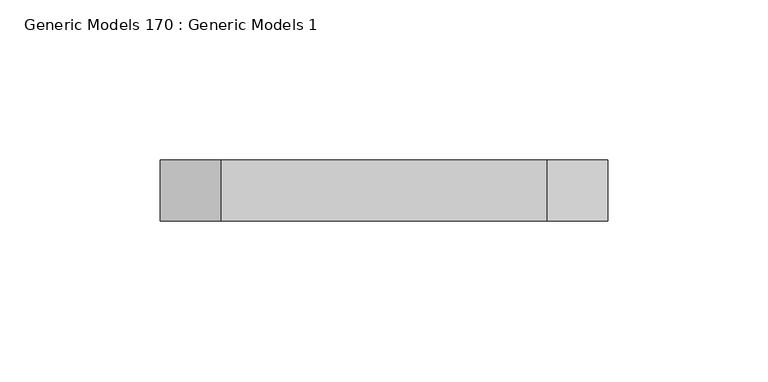
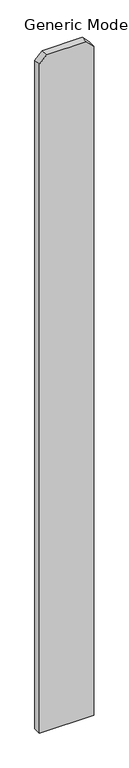
"""IFC4 building model written with IfcOpenShell, lengths in millimetres: proxy geometry, Generic Models 170 : Generic Models 1."""

import ifcopenshell
import ifcopenshell.guid

model = None  # the IFC model being written
_history = None  # IfcOwnerHistory: only IFC2X3 demands one
_inside = {}  # id of a spatial element -> (the spatial element, [elements in it])
_under = {}  # id of a project, library or spatial element -> (it, [spatial elements below it])
_declared = {}  # id of a project -> (the project, [libraries it declares])
_typed = {}  # id of a type object -> (the type object, [elements of that type])
_made_of = {}  # id of a material, layer set ... -> (it, [elements and type objects made of it])


def new_model(schema):
    """Start an empty IFC model of exactly this schema.

    Asked for "IFC4X3", IfcOpenShell would pick the latest addendum, in which some entities
    have other attributes; the version numbers below select the first issue.
    IFC2X3 requires an IfcOwnerHistory on every rooted entity: one is made here for all.
    """
    global model, _history
    if schema == "IFC4X3":
        model = ifcopenshell.file(schema_version=(4, 3, 0, 0))
    else:
        model = ifcopenshell.file(schema=schema)
    _inside.clear()
    _under.clear()
    _declared.clear()
    _typed.clear()
    _made_of.clear()
    _history = None
    if model.schema == "IFC2X3":
        org = make("IfcOrganization", Name="unknown")
        user = make(
            "IfcPersonAndOrganization",
            ThePerson=make("IfcPerson", FamilyName="unknown"),
            TheOrganization=org,
        )
        app = make(
            "IfcApplication",
            ApplicationDeveloper=org,
            Version="unknown",
            ApplicationFullName="unknown",
            ApplicationIdentifier="unknown",
        )
        _history = make(
            "IfcOwnerHistory",
            OwningUser=user,
            OwningApplication=app,
            ChangeAction="ADDED",
            CreationDate=0,
        )
    return model


def make(cls, **values):
    """One entity of the class cls with the attributes given. An attribute that is None is left unset."""
    return model.create_entity(
        cls, **{name: value for name, value in values.items() if value is not None}
    )


def rooted(cls, **values):
    """An entity with a GlobalId (a new one), such as an element, a storey or a relation."""
    return make(cls, GlobalId=ifcopenshell.guid.new(), OwnerHistory=_history, **values)


def si_unit(unit_type, name, prefix=None):
    """IfcSIUnit, for example si_unit("LENGTHUNIT", "METRE", prefix="MILLI")."""
    return make("IfcSIUnit", UnitType=unit_type, Prefix=prefix, Name=name)


def assignment(units):
    """IfcUnitAssignment: the units of a project."""
    return None if units is None else make("IfcUnitAssignment", Units=units)


def point(xyz):
    """IfcCartesianPoint."""
    return None if xyz is None else make("IfcCartesianPoint", Coordinates=xyz)


def direction(xyz):
    """IfcDirection."""
    return None if xyz is None else make("IfcDirection", DirectionRatios=xyz)


def frame(location, z_axis=None, x_axis=None):
    """IfcAxis2Placement3D, a coordinate frame: its origin and axes. An axis left out is left unset."""
    return make(
        "IfcAxis2Placement3D",
        Location=point(location),
        Axis=direction(z_axis),
        RefDirection=direction(x_axis),
    )


def origin():
    """The frame at (0, 0, 0) with its axes left unset."""
    return frame((0.0, 0.0, 0.0))


def place(relative_to, where):
    """IfcLocalPlacement: puts the frame where relative to a parent placement (None: the world)."""
    return make(
        "IfcLocalPlacement", PlacementRelTo=relative_to, RelativePlacement=where
    )


def context(
    kind, dimensions, precision=None, world=None, true_north=None, identifier=None
):
    """IfcGeometricRepresentationContext, for example the 3D "Model" context."""
    return make(
        "IfcGeometricRepresentationContext",
        ContextIdentifier=identifier,
        ContextType=kind,
        CoordinateSpaceDimension=dimensions,
        Precision=precision,
        WorldCoordinateSystem=world,
        TrueNorth=true_north,
    )


def project(units=None, contexts=None):
    """IfcProject with its units and contexts."""
    return rooted(
        "IfcProject",
        Name="project",
        RepresentationContexts=contexts,
        UnitsInContext=assignment(units),
    )


def spatial(cls, under=None, at=None, **own):
    """A site, building, storey or space (cls), placed at a placement, below another one or the project."""
    s = rooted(cls, ObjectPlacement=at, **own)
    if under is not None:
        _under.setdefault(under.id(), (under, []))[1].append(s)
    return s


def polyline(points):
    """IfcPolyline through the points."""
    return make("IfcPolyline", Points=[point(p) for p in points])


def outline(outer, holes=None, kind="AREA"):
    """IfcArbitraryClosedProfileDef: a profile drawn as a closed curve; with holes, ...WithVoids."""
    if holes is None:
        return make("IfcArbitraryClosedProfileDef", ProfileType=kind, OuterCurve=outer)
    return make(
        "IfcArbitraryProfileDefWithVoids",
        ProfileType=kind,
        OuterCurve=outer,
        InnerCurves=holes,
    )


def extrude(swept, where, along, depth):
    """IfcExtrudedAreaSolid: the profile swept, set in the frame where, extruded along a direction by depth."""
    return make(
        "IfcExtrudedAreaSolid",
        SweptArea=swept,
        Position=where,
        ExtrudedDirection=direction(along),
        Depth=depth,
    )


def shape(context_of_items, identifier, shape_type, items):
    """IfcShapeRepresentation: the items that make up one representation, for example the "Body"."""
    return make(
        "IfcShapeRepresentation",
        ContextOfItems=context_of_items,
        RepresentationIdentifier=identifier,
        RepresentationType=shape_type,
        Items=items,
    )


def source(mapping_origin, context_of_items, identifier, shape_type, items):
    """IfcRepresentationMap: a shape defined once, which mapped items show again and again."""
    return make(
        "IfcRepresentationMap",
        MappingOrigin=mapping_origin,
        MappedRepresentation=shape(context_of_items, identifier, shape_type, items),
    )


def transform(
    local_origin,
    x_axis=None,
    y_axis=None,
    z_axis=None,
    scale=None,
    scale2=None,
    scale3=None,
    uniform=True,
):
    """IfcCartesianTransformationOperator3D, or its non-uniform kind. x_axis, y_axis, z_axis: its Axis1, 2, 3."""
    if uniform:
        return make(
            "IfcCartesianTransformationOperator3D",
            Axis1=direction(x_axis),
            Axis2=direction(y_axis),
            LocalOrigin=point(local_origin),
            Scale=scale,
            Axis3=direction(z_axis),
        )
    return make(
        "IfcCartesianTransformationOperator3DnonUniform",
        Axis1=direction(x_axis),
        Axis2=direction(y_axis),
        LocalOrigin=point(local_origin),
        Scale=scale,
        Axis3=direction(z_axis),
        Scale2=scale2,
        Scale3=scale3,
    )


def mapped(mapping_source, mapping_target):
    """IfcMappedItem: shows the shape of a source again, moved by a transform."""
    return make(
        "IfcMappedItem", MappingSource=mapping_source, MappingTarget=mapping_target
    )


def made_of(thing, what):
    """Note that an element or type object is made of a material, layer set ...; save() writes the relation."""
    if what is not None:
        _made_of.setdefault(what.id(), (what, []))[1].append(thing)
    return thing


def element(
    cls,
    number,
    at=None,
    inside=None,
    cuts=None,
    type_object=None,
    material=None,
    context=None,
    identifier="Body",
    shape_type=None,
    held_by="IfcProductDefinitionShape",
    body=None,
    shapes=None,
    **own,
):
    """One element of the class cls, such as IfcWall. Its Tag is "e" and its number.

    at: its placement. inside: the storey or other place that contains it. cuts: it is an
    opening in that element (IfcRelVoidsElement). A single representation is given by context,
    identifier, shape_type and body (its items); several are given by shapes. held_by: the class
    of the entity that holds the representations. save() writes the other relations.
    """
    e = rooted(cls, Tag="e%d" % number, ObjectPlacement=at, **own)
    if body is not None:
        shapes = [shape(context, identifier, shape_type, body)]
    if shapes is not None:
        e.Representation = make(held_by, Representations=shapes)
    if inside is not None:
        _inside.setdefault(inside.id(), (inside, []))[1].append(e)
    if cuts is not None:
        rooted(
            "IfcRelVoidsElement", RelatingBuildingElement=cuts, RelatedOpeningElement=e
        )
    if type_object is not None:
        _typed.setdefault(type_object.id(), (type_object, []))[1].append(e)
    return made_of(e, material)


def aggregate(whole, parts):
    """IfcRelAggregates: a whole, such as a stair, and the parts it consists of."""
    return rooted("IfcRelAggregates", RelatingObject=whole, RelatedObjects=parts)


def save(model, path):
    """Write the relations noted so far, then the file.

    IfcRelAggregates (storeys below a building ...), IfcRelContainedInSpatialStructure (elements
    in a storey), IfcRelDefinesByType, IfcRelAssociatesMaterial and IfcRelDeclares: one each for
    every whole, place, type object, material and project.
    """
    for whole, parts in _under.values():
        aggregate(whole, parts)
    for where, things in _inside.values():
        rooted(
            "IfcRelContainedInSpatialStructure",
            RelatedElements=things,
            RelatingStructure=where,
        )
    for kind, things in _typed.values():
        rooted("IfcRelDefinesByType", RelatedObjects=things, RelatingType=kind)
    for what, things in _made_of.values():
        rooted("IfcRelAssociatesMaterial", RelatedObjects=things, RelatingMaterial=what)
    for by, libraries in _declared.values():
        rooted("IfcRelDeclares", RelatingContext=by, RelatedDefinitions=libraries)
    model.write(path)


def generic_models_170_generic_models_1_1b954c43(model_context):
    return source(origin(), model_context, "Body", "SweptSolid", [
        extrude(outline(polyline([(76.2, 55903.8125), (1885.95, 55903.8125), (1905.0, 55884.7625), (1905.0, 55783.1625), (1885.95, 55764.1125), (76.2, 55764.1125), (76.2, 55903.8125)])), frame((0.0, 547.6875, 0.0), z_axis=(0.0, 1.0, 0.0), x_axis=(0.0, 0.0, 1.0)), (0.0, 0.0, 1.0), 19.05),
    ])


if __name__ == "__main__":
    model = new_model("IFC4")
    model_context = context("Model", 3, world=origin())
    ifc_project = project(units=[si_unit("LENGTHUNIT", "METRE", prefix="MILLI")], contexts=[model_context])
    site = spatial("IfcSite", under=ifc_project)
    building = spatial("IfcBuilding", under=site)
    placement = place(None, origin())
    generic_models_170_generic_models_1_shape = generic_models_170_generic_models_1_1b954c43(model_context)
    element("IfcBuildingElementProxy", 1, Name="Generic Models 170 : Generic Models 1", ObjectType="Generic Models 170 : Generic Models 1", at=placement, inside=building, context=model_context, shape_type="MappedRepresentation", body=[
        mapped(generic_models_170_generic_models_1_shape, transform((0.0, 0.0, 0.0), x_axis=(1.0, 0.0, 0.0), y_axis=(0.0, 1.0, 0.0), z_axis=(0.0, 0.0, 1.0))),
    ])
    save(model, "model.ifc")

# Revit data of these elements
# Project information
#   Project Issue Date = "09/11/2018"
#   Project Status = "Project Status"
#   Client Name = "Owner"
#   Project Address = "1021 HIGH ST -  MADISON, WI 53715"
#   Project Name = "2ND FLOOR ADDITION"
#   Project Number = "Project Number"
# Element 1 (IfcBuildingElementProxy, "Generic Models 170 : Generic Models 1")
#   Materials on its faces: "VERTICAL 1X6 CEDAR PLANKS W/ CLEAR WOOD SEALER"
# Materials
#   "VERTICAL 1X6 CEDAR PLANKS W/ CLEAR WOOD SEALER": class "Wood", colour RGB 234 198 147, transparency 0, Description = "Pinus Echinata", Cost = 0
